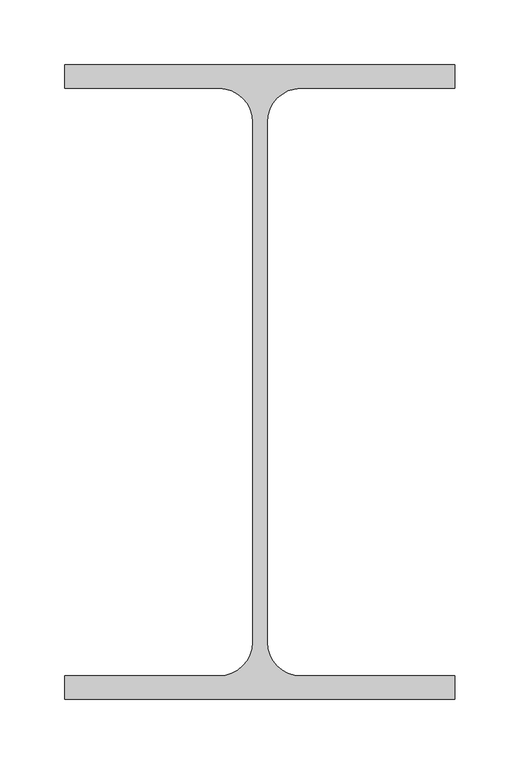
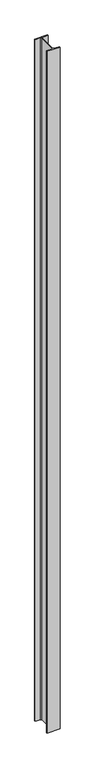
"""IFC4 building model written with IfcOpenShell, lengths in millimetres: column geometry, 0912_Steel Column_H_KSD3502 : H_SC_ASC_H-488x300x11x18."""

from ifc_helpers import new_model, si_unit, point, frame, frame_2d, origin, place, context, project, spatial, polyline, circle_curve, trimmed, segment, composite_curve, outline, extrude, source, transform, mapped, element, save


def column_8b02a347(model_context):
    return source(origin(), model_context, "Body", "SweptSolid", [
        extrude(outline(composite_curve([segment(polyline([(150.0, 244.0), (150.0, 226.0), (31.5, 226.0)]), True, "CONTINUOUS"), segment(trimmed(circle_curve(frame_2d((31.5, 200.0)), 26.0), [point((31.5, 226.0))], [point((5.5, 200.0))], True, "CARTESIAN"), True, "CONTINUOUS"), segment(polyline([(5.5, 200.0), (5.5, -200.0)]), True, "CONTINUOUS"), segment(trimmed(circle_curve(frame_2d((31.5, -200.0)), 26.0), [point((5.5, -200.0))], [point((31.5, -226.0))], True, "CARTESIAN"), True, "CONTINUOUS"), segment(polyline([(31.5, -226.0), (150.0, -226.0), (150.0, -244.0), (-150.0, -244.0), (-150.0, -226.0), (-31.5, -226.0)]), True, "CONTINUOUS"), segment(trimmed(circle_curve(frame_2d((-31.5, -200.0)), 26.0), [point((-31.5, -226.0))], [point((-5.5, -200.0))], True, "CARTESIAN"), True, "CONTINUOUS"), segment(polyline([(-5.5, -200.0), (-5.5, 200.0)]), True, "CONTINUOUS"), segment(trimmed(circle_curve(frame_2d((-31.5, 200.0)), 26.0), [point((-5.5, 200.0))], [point((-31.5, 226.0))], True, "CARTESIAN"), True, "CONTINUOUS"), segment(polyline([(-31.5, 226.0), (-150.0, 226.0), (-150.0, 244.0), (150.0, 244.0)]), True, "CONTINUOUS")], self_intersect=False)), frame((0.0, 0.0, 685.9720055), z_axis=(0.0, 0.0, 1.0), x_axis=(1.0, 0.0, 0.0)), (0.0, 0.0, 1.0), 16614.0),
    ])


if __name__ == "__main__":
    model = new_model("IFC4")
    model_context = context("Model", 3, world=origin())
    ifc_project = project(units=[si_unit("LENGTHUNIT", "METRE", prefix="MILLI")], contexts=[model_context])
    site = spatial("IfcSite", under=ifc_project)
    building = spatial("IfcBuilding", under=site)
    placement = place(None, origin())
    column_shape = column_8b02a347(model_context)
    element("IfcColumn", 1, ObjectType="0912_Steel Column_H_KSD3502 : H_SC_ASC_H-488x300x11x18", at=placement, inside=building, context=model_context, shape_type="MappedRepresentation", body=[
        mapped(column_shape, transform((0.0, 0.0, 0.0), x_axis=(1.0, 0.0, 0.0), y_axis=(0.0, 1.0, 0.0), z_axis=(0.0, 0.0, 1.0))),
    ])
    save(model, "model.ifc")

# Revit data of these elements
# Type "0912_Steel Column_H_KSD3502 : H_SC_ASC_H-488x300x11x18"
#   H_WM Code_1 = "S01AA002-00001 | Main Steel Structure Fabrication Work | Shelter/Building | Medium Steel - Standard (90KG/M>Weight≥30KG/M) | Material: (   )"
#   H_WM Code_2 = "S03AA028-00001 | Main Steel Structure Erection Work | Shelter/Building | Medium Steel (90KG/M>Weight≥30KG/M) | Material: (   )"
#   H_WM Code_3 = "S01AA010-00001 | Main Steel Structure Fabrication Work | Shelter/Building | Steel Painting/Coating | for Non-Fireproofed Steel Surface, Surface Preparation, Primer, Second & Final Coat | Material: (   )"
#   H_Q'ty Cal Type Tag = "SC-Q2"
#   Width = 30.0 cm
#   Web Thickness = 1.1 cm
#   Web Fillet = 2.6 cm
#   Warping Constant = 4473230.0 cm⁶
#   Torsional Moment of Inertia = 137.492 cm⁴
#   Section Area = 163.5 cm²
#   Plastic Modulus weak axis = 830.0 cm³
#   Plastic Modulus strong axis = 3230.0 cm³
#   Perimeter = 2.11 m²/m
#   Nominal Weight = 128.00 kgf/m
#   Moment of Inertia weak axis = 8110.00 cm⁴
#   Moment of Inertia strong axis = 71000.00 cm⁴
#   Height = 48.8 cm
#   Flange Thickness = 1.8 cm
#   Elastic Modulus weak axis = 541.0 cm³
#   Elastic Modulus strong axis = 2910.0 cm³
#   Centroid Vertical = 24.4 cm
#   Centroid Horizontal = 15.0 cm
#   Structural Material [instance default] = Steel, 45-345
#   Section Name Key = ""
#   Bolt Spacing = 0
#   Assembly Code = ""
# Element 1 (IfcColumn, "0912_Steel Column_H_KSD3502 : H_SC_ASC_H-488x300x11x18")
#   Structural Material = A03AD029-00005_Anchor Bolt (Installation only)_M24
#   Materials on its faces: "A03AD029-00005_Anchor Bolt (Installation only)_M24"
# Materials
#   "Steel, 45-345": class "Metal", colour RGB 189 187 185, transparency 0, Description = "Steel 345 MPa", Cost = 0
#   "A03AD029-00005_Anchor Bolt (Installation only)_M24": class "Unassigned", colour RGB 84 83 81, transparency 0, Cost = 0
